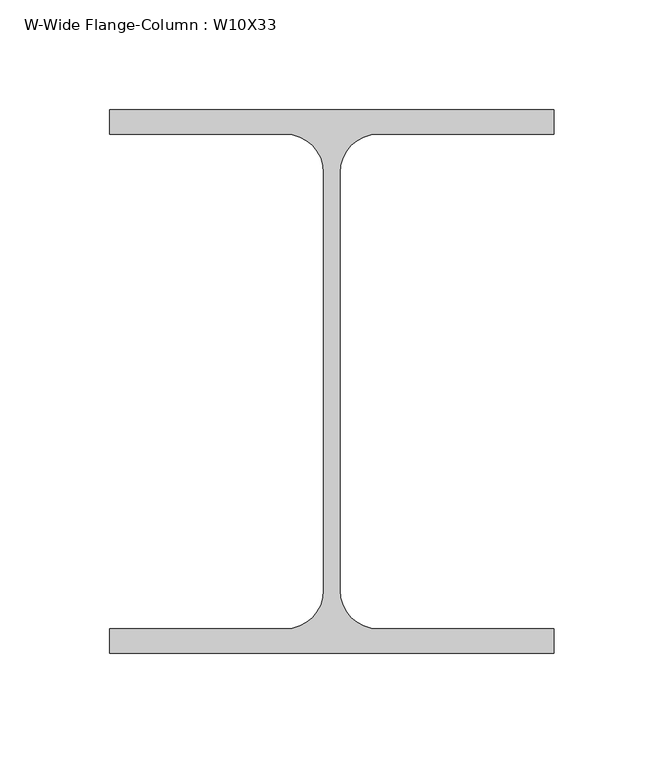
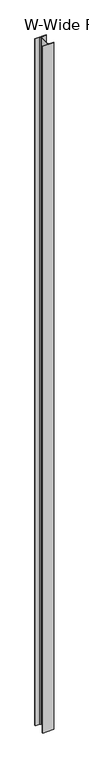
"""IFC4 building model written with IfcOpenShell, lengths in millimetres: column geometry, W-Wide Flange-Column : W10X33."""

from ifc_helpers import new_model, si_unit, point, frame, frame_2d, origin, place, context, project, spatial, polyline, circle_curve, trimmed, segment, composite_curve, outline, extrude, source, transform, mapped, element, save


def w_wide_flange_column_w10x33_ab5edc20(model_context):
    return source(origin(), model_context, "Body", "SweptSolid", [
        extrude(outline(composite_curve([segment(polyline([(101.092, 123.571), (101.092, 112.522), (21.209, 112.522)]), True, "CONTINUOUS"), segment(trimmed(circle_curve(frame_2d((21.209, 94.996)), 17.526), [point((21.209, 112.522))], [point((3.683, 94.996))], True, "CARTESIAN"), True, "CONTINUOUS"), segment(polyline([(3.683, 94.996), (3.683, -94.996)]), True, "CONTINUOUS"), segment(trimmed(circle_curve(frame_2d((21.209, -94.996)), 17.526), [point((3.683, -94.996))], [point((21.209, -112.522))], True, "CARTESIAN"), True, "CONTINUOUS"), segment(polyline([(21.209, -112.522), (101.092, -112.522), (101.092, -123.571), (-101.092, -123.571), (-101.092, -112.522), (-21.209, -112.522)]), True, "CONTINUOUS"), segment(trimmed(circle_curve(frame_2d((-21.209, -94.996)), 17.526), [point((-21.209, -112.522))], [point((-3.683, -94.996))], True, "CARTESIAN"), True, "CONTINUOUS"), segment(polyline([(-3.683, -94.996), (-3.683, 94.996)]), True, "CONTINUOUS"), segment(trimmed(circle_curve(frame_2d((-21.209, 94.996)), 17.526), [point((-3.683, 94.996))], [point((-21.209, 112.522))], True, "CARTESIAN"), True, "CONTINUOUS"), segment(polyline([(-21.209, 112.522), (-101.092, 112.522), (-101.092, 123.571), (101.092, 123.571)]), True, "CONTINUOUS")], self_intersect=False)), frame((0.0, 0.0, 8756.65), z_axis=(0.0, 0.0, 1.0), x_axis=(1.0, 0.0, 0.0)), (0.0, 0.0, 1.0), 13138.15),
    ])


if __name__ == "__main__":
    model = new_model("IFC4")
    model_context = context("Model", 3, world=origin())
    ifc_project = project(units=[si_unit("LENGTHUNIT", "METRE", prefix="MILLI")], contexts=[model_context])
    site = spatial("IfcSite", under=ifc_project)
    building = spatial("IfcBuilding", under=site)
    placement = place(None, origin())
    w_wide_flange_column_w10x33_shape = w_wide_flange_column_w10x33_ab5edc20(model_context)
    element("IfcColumn", 1, ObjectType="W-Wide Flange-Column : W10X33", at=placement, inside=building, context=model_context, shape_type="MappedRepresentation", body=[
        mapped(w_wide_flange_column_w10x33_shape, transform((0.0, 0.0, 0.0), x_axis=(1.0, 0.0, 0.0), y_axis=(0.0, 1.0, 0.0), z_axis=(0.0, 0.0, 1.0))),
    ])
    save(model, "model.ifc")

# Revit data of these elements
# Type "W-Wide Flange-Column : W10X33"
#   Assembly Code = "B10"
#   W = 33
#   bf = 0' - 7.96"
#   d = 0' - 9.73"
#   k = 0' - 1 1/8"
#   kr = 0' - 0.69"
#   tf = 0' - 0.435"
#   tw = 0' - 0.29"
#   A = 0.0674306 SF
#   Structural Material [instance default] = Steel ASTM A992
# Element 1 (IfcColumn, "W-Wide Flange-Column : W10X33")
#   Materials on its faces: "Steel ASTM A992"
# Materials
#   "Steel ASTM A992": class "Metal", colour RGB 199 199 199, transparency 0, Description = "Structural steel 50ksi", Cost = 0
